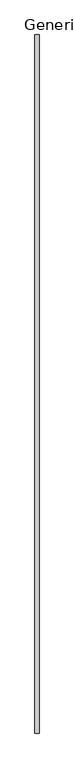
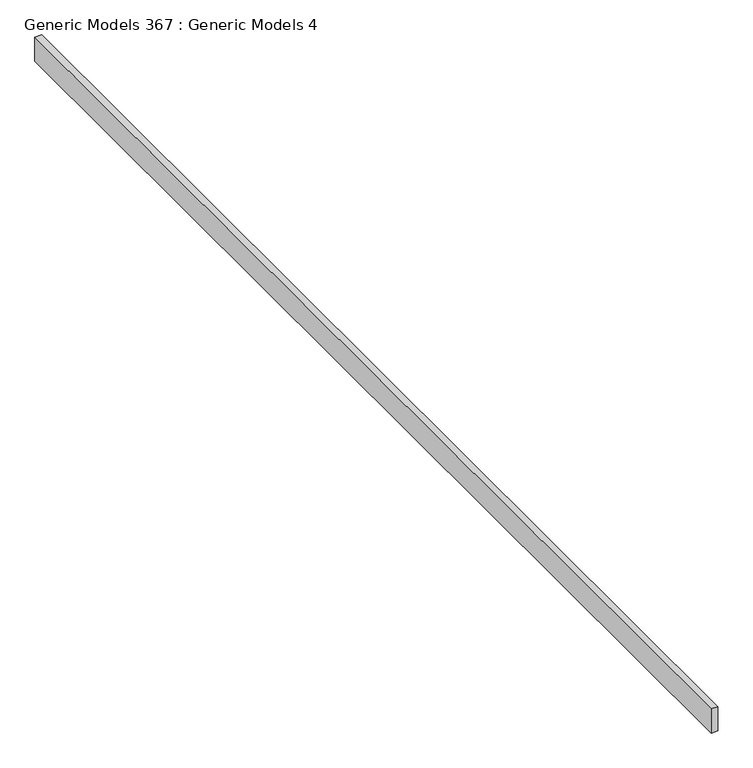
"""IFC4 building model written with IfcOpenShell, lengths in millimetres: proxy geometry, Generic Models 367 : Generic Models 4."""

from ifc_helpers import new_model, si_unit, frame, origin, place, context, project, spatial, polyline, outline, extrude, source, transform, mapped, element, save


def generic_models_367_generic_models_4_ffb0c3c9(model_context):
    return source(origin(), model_context, "Body", "SweptSolid", [
        extrude(outline(polyline([(-6521.6236296, -6864.9230338), (-6559.7236296, -6864.9230338), (-6559.7236296, -464.1230338), (-6521.6236296, -464.1230338), (-6521.6236296, -6864.9230338)])), frame((0.0, 0.0, 129093.3123933), z_axis=(0.0, 0.0, 1.0), x_axis=(1.0, 0.0, 0.0)), (0.0, 0.0, 1.0), 139.7),
    ])


if __name__ == "__main__":
    model = new_model("IFC4")
    model_context = context("Model", 3, world=origin())
    ifc_project = project(units=[si_unit("LENGTHUNIT", "METRE", prefix="MILLI")], contexts=[model_context])
    site = spatial("IfcSite", under=ifc_project)
    building = spatial("IfcBuilding", under=site)
    placement = place(None, origin())
    generic_models_367_generic_models_4_shape = generic_models_367_generic_models_4_ffb0c3c9(model_context)
    element("IfcBuildingElementProxy", 1, Name="Generic Models 367 : Generic Models 4", ObjectType="Generic Models 367 : Generic Models 4", at=placement, inside=building, context=model_context, shape_type="MappedRepresentation", body=[
        mapped(generic_models_367_generic_models_4_shape, transform((0.0, 0.0, 0.0), x_axis=(1.0, 0.0, 0.0), y_axis=(0.0, 1.0, 0.0), z_axis=(0.0, 0.0, 1.0))),
    ])
    save(model, "model.ifc")

# Revit data of these elements
# Element 1 (IfcBuildingElementProxy, "Generic Models 367 : Generic Models 4")
#   Materials on its faces: "_2X BLOCKING AS REQUIRED"
# Materials
#   "_2X BLOCKING AS REQUIRED": class "Generic", colour RGB 177 130 114, transparency 0, Cost = 0
